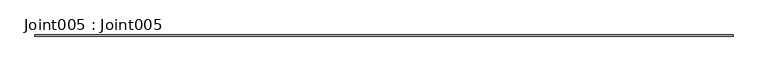
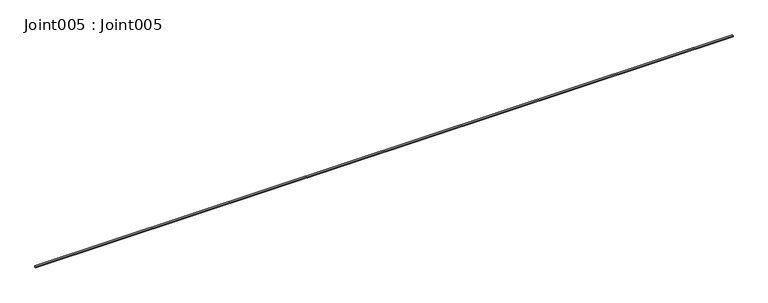
"""IFC4 building model written with IfcOpenShell, lengths in millimetres: proxy geometry, Joint005 : Joint005."""

from ifc_helpers import new_model, si_unit, point, frame, frame_2d, origin, place, context, project, spatial, polyline, circle_curve, trimmed, segment, composite_curve, outline, extrude, source, transform, mapped, element, save


def joint005_joint005_2fc430ad(model_context):
    return source(origin(), model_context, "Body", "SweptSolid", [
        extrude(outline(composite_curve([segment(polyline([(10407.9541245, 42894.7389688), (10407.9541245, 42890.821)]), True, "CONTINUOUS"), segment(trimmed(circle_curve(frame_2d((10406.3557924, 42885.649125)), 5.4132205), [point((10407.9541245, 42890.821))], [point((10404.7574604, 42890.821))], True, "CARTESIAN"), True, "CONTINUOUS"), segment(polyline([(10404.7574604, 42890.821), (10404.7574604, 42894.7389688)]), True, "CONTINUOUS"), segment(trimmed(circle_curve(frame_2d((10406.3557924, 42889.5670938)), 5.4132205), [point((10404.7574604, 42894.7389688))], [point((10407.9541245, 42894.7389688))], False, "CARTESIAN"), True, "CONTINUOUS")], self_intersect=False)), frame((3694.2883192, 0.0, 0.0), z_axis=(1.0, 0.0, 0.0), x_axis=(0.0, 1.0, 0.0)), (0.0, 0.0, 1.0), 2000.0),
    ])


if __name__ == "__main__":
    model = new_model("IFC4")
    model_context = context("Model", 3, world=origin())
    ifc_project = project(units=[si_unit("LENGTHUNIT", "METRE", prefix="MILLI")], contexts=[model_context])
    site = spatial("IfcSite", under=ifc_project)
    building = spatial("IfcBuilding", under=site)
    placement = place(None, origin())
    joint005_joint005_shape = joint005_joint005_2fc430ad(model_context)
    element("IfcBuildingElementProxy", 1, Name="Joint005 : Joint005", ObjectType="Joint005 : Joint005", at=placement, inside=building, context=model_context, shape_type="MappedRepresentation", body=[
        mapped(joint005_joint005_shape, transform((0.0, 0.0, 0.0), x_axis=(1.0, 0.0, 0.0), y_axis=(0.0, 1.0, 0.0), z_axis=(0.0, 0.0, 1.0))),
    ])
    save(model, "model.ifc")

# Revit data of these elements
# Type "Joint005 : Joint005"
#   NameOverride = "Joint005"
# Element 1 (IfcBuildingElementProxy, "Joint005 : Joint005")
#   Materials on its faces: "SEALANT JOINT"
# Materials
#   "SEALANT JOINT": class "Unassigned", colour RGB 142 225 148, transparency 0
